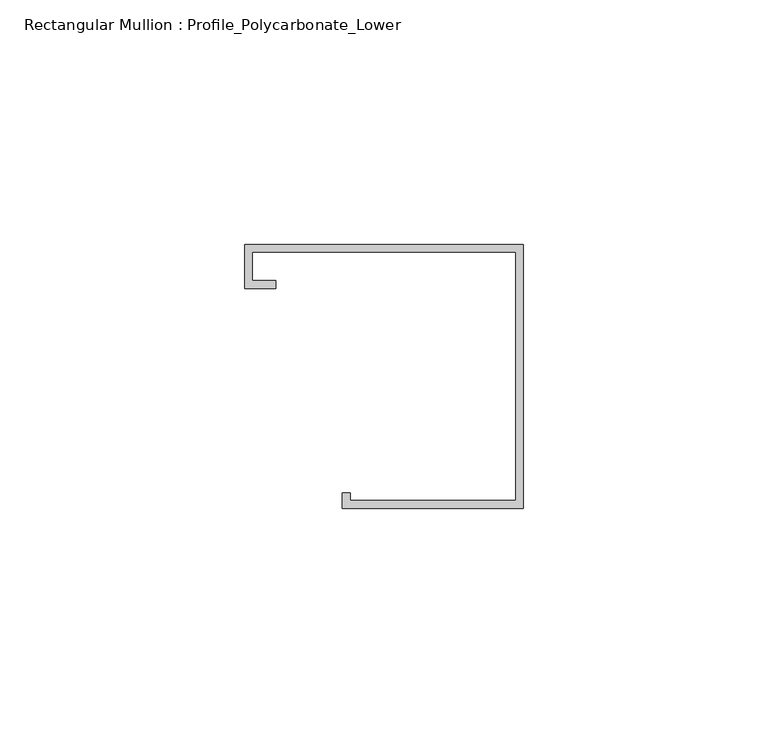
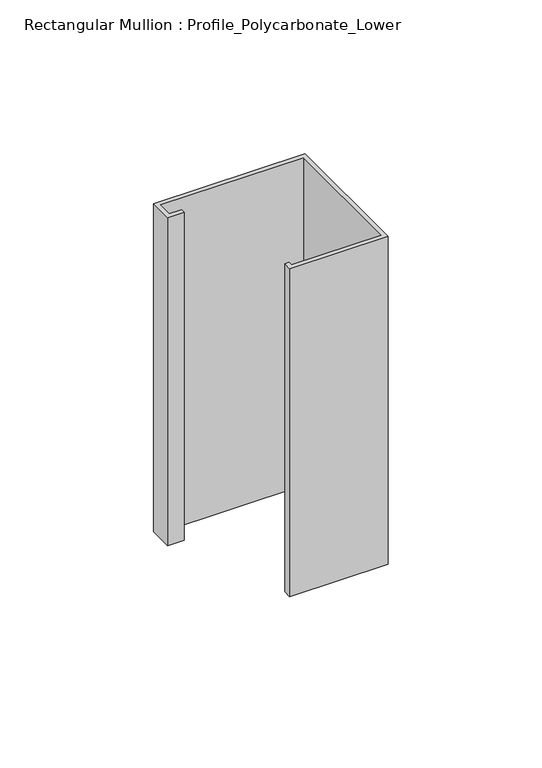
"""IFC4 building model written with IfcOpenShell, lengths in millimetres: member geometry, Rectangular Mullion : Profile_Polycarbonate_Lower."""

from ifc_helpers import new_model, si_unit, frame, origin, place, context, project, spatial, polyline, outline, extrude, source, transform, mapped, element, save


def rectangular_mullion_profile_polycarbonate_lower_cc0376f6(model_context):
    return source(origin(), model_context, "Body", "SweptSolid", [
        extrude(outline(polyline([(0.0, 28.984575), (0.0, -25.015825), (-36.9824, -25.015825), (-36.9824, -21.840825), (-35.3949, -21.840825), (-35.3949, -23.428325), (-1.5875, -23.428325), (-1.5875, 27.397075), (-55.4101, 27.397075), (-55.4101, 21.580475), (-50.6476, 21.580475), (-50.6476, 19.992975), (-56.9976, 19.992975), (-56.9976, 28.984575), (0.0, 28.984575)])), frame((0.0, 0.0, -130.2512), z_axis=(0.0, 0.0, 1.0), x_axis=(1.0, 0.0, 0.0)), (0.0, 0.0, 1.0), 130.2512),
    ])


if __name__ == "__main__":
    model = new_model("IFC4")
    model_context = context("Model", 3, world=origin())
    ifc_project = project(units=[si_unit("LENGTHUNIT", "METRE", prefix="MILLI")], contexts=[model_context])
    site = spatial("IfcSite", under=ifc_project)
    building = spatial("IfcBuilding", under=site)
    placement = place(None, origin())
    rectangular_mullion_profile_polycarbonate_lower_shape = rectangular_mullion_profile_polycarbonate_lower_cc0376f6(model_context)
    element("IfcMember", 1, ObjectType="Rectangular Mullion : Profile_Polycarbonate_Lower", at=placement, inside=building, context=model_context, shape_type="MappedRepresentation", body=[
        mapped(rectangular_mullion_profile_polycarbonate_lower_shape, transform((0.0, 0.0, 0.0), x_axis=(1.0, 0.0, 0.0), y_axis=(0.0, 1.0, 0.0), z_axis=(0.0, 0.0, 1.0))),
    ])
    save(model, "model.ifc")

# Revit data of these elements
# Type "Rectangular Mullion : Profile_Polycarbonate_Lower"
#   built-in parameter 1007322 = 0.177167 (stored number, unit not read)
#   built-in parameter 1007321 = 0 (stored number, unit not read)
#   built-in parameter 1007320 = 0.00520833 (stored number, unit not read)
